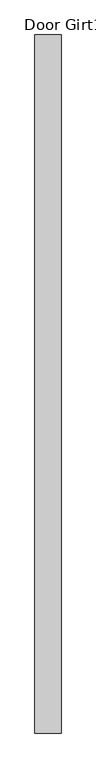
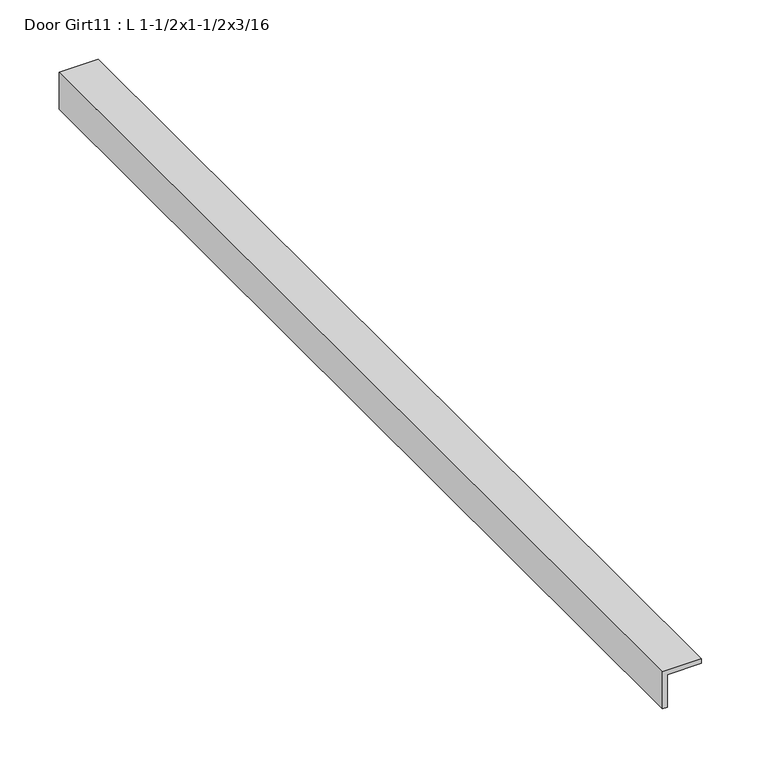
"""IFC4 building model written with IfcOpenShell, lengths in millimetres: proxy geometry, Door Girt11 : L 1-1/2x1-1/2x3/16."""

from ifc_helpers import new_model, si_unit, frame, origin, place, context, project, spatial, polyline, outline, extrude, source, transform, mapped, element, save


def door_girt11_l_1_1_2x1_1_2x3_16_9aa2a562(model_context):
    return source(origin(), model_context, "Body", "SweptSolid", [
        extrude(outline(polyline([(812.8, 587403.9934739), (812.8, 587365.8934739), (774.7, 587365.8934739), (774.7, 587370.6559739), (808.0375, 587370.6559739), (808.0375, 587403.9934739), (812.8, 587403.9934739)])), frame((0.0, -536263.6038841, 0.0), z_axis=(0.0, 1.0, 0.0), x_axis=(0.0, 0.0, 1.0)), (0.0, 0.0, 1.0), 1017.5875),
    ])


if __name__ == "__main__":
    model = new_model("IFC4")
    model_context = context("Model", 3, world=origin())
    ifc_project = project(units=[si_unit("LENGTHUNIT", "METRE", prefix="MILLI")], contexts=[model_context])
    site = spatial("IfcSite", under=ifc_project)
    building = spatial("IfcBuilding", under=site)
    placement = place(None, origin())
    door_girt11_l_1_1_2x1_1_2x3_16_shape = door_girt11_l_1_1_2x1_1_2x3_16_9aa2a562(model_context)
    element("IfcBuildingElementProxy", 1, Name="Door Girt11 : L 1-1/2x1-1/2x3/16", ObjectType="Door Girt11 : L 1-1/2x1-1/2x3/16", at=placement, inside=building, context=model_context, shape_type="MappedRepresentation", body=[
        mapped(door_girt11_l_1_1_2x1_1_2x3_16_shape, transform((0.0, 0.0, 0.0), x_axis=(1.0, 0.0, 0.0), y_axis=(0.0, 1.0, 0.0), z_axis=(0.0, 0.0, 1.0))),
    ])
    save(model, "model.ifc")

# Revit data of these elements
# Element 1 (IfcBuildingElementProxy, "Door Girt11 : L 1-1/2x1-1/2x3/16")
#   Materials on its faces: "1-1/2\"X1-1/2\" GALV. STL L"
# Materials
#   "1-1/2\"X1-1/2\" GALV. STL L": class "Generic", colour RGB 211 211 207, transparency 0, Cost = 0
